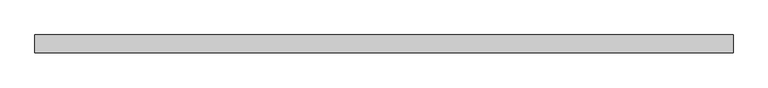
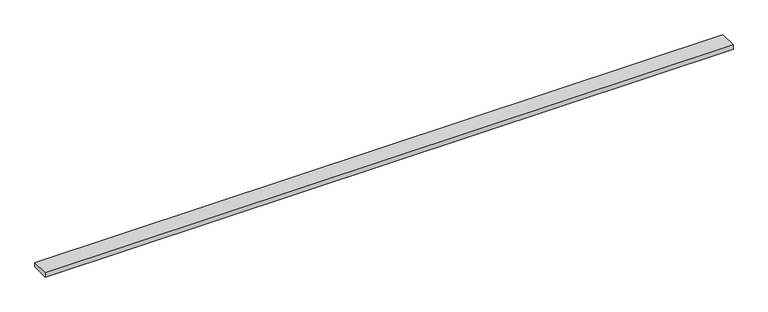
"""IFC4 building model written with IfcOpenShell, lengths in millimetres: proxy geometry, Generic Models 6:Generic Models 2:318829:Generic Models 2:318829 : Generic Models 6:Generic Models 2:318829:20 : Generic Models 6:Generic Models 2:318829:Generic Models 2:318829 : Generic Models 6:Generic Models 2:318829:300683."""

from ifc_helpers import new_model, si_unit, frame, origin, place, context, project, spatial, polyline, outline, extrude, source, transform, mapped, element, save


def generic_models_66336ed3(model_context):
    return source(origin(), model_context, "Body", "SweptSolid", [
        extrude(outline(polyline([(592755.4242239, -579000.6913841), (592755.4242239, -579063.015441), (590317.0242239, -579063.015441), (590317.0242239, -579000.6913841), (592755.4242239, -579000.6913841)])), frame((0.0, 0.0, 3699.7749221), z_axis=(0.0, 0.0, 1.0), x_axis=(1.0, 0.0, 0.0)), (0.0, 0.0, 1.0), 15.837253),
    ])


if __name__ == "__main__":
    model = new_model("IFC4")
    model_context = context("Model", 3, world=origin())
    ifc_project = project(units=[si_unit("LENGTHUNIT", "METRE", prefix="MILLI")], contexts=[model_context])
    site = spatial("IfcSite", under=ifc_project)
    building = spatial("IfcBuilding", under=site)
    placement = place(None, origin())
    generic_models_shape = generic_models_66336ed3(model_context)
    element("IfcBuildingElementProxy", 1, Name="Generic Models 6:Generic Models 2:318829:Generic Models 2:318829 : Generic Models 6:Generic Models 2:318829:20 : Generic Models 6:Generic Models 2:318829:Generic Models 2:318829 : Generic Models 6:Generic Models 2:318829:300683", ObjectType="Generic Models 6:Generic Models 2:318829:Generic Models 2:318829 : Generic Models 6:Generic Models 2:318829:20 : Generic Models 6:Generic Models 2:318829:Generic Models 2:318829 : Generic Models 6:Generic Models 2:318829:300683", at=placement, inside=building, context=model_context, shape_type="MappedRepresentation", body=[
        mapped(generic_models_shape, transform((0.0, 0.0, 0.0), x_axis=(1.0, 0.0, 0.0), y_axis=(0.0, 1.0, 0.0), z_axis=(0.0, 0.0, 1.0))),
    ])
    save(model, "model.ifc")

# Revit data of these elements
# Type "Generic Models 6:Generic Models 2:318829:Generic Models 2:318829 : Generic Models 6:Generic Models 2:318829:20 : Generic Models 6:Generic Models 2:318829:Generic Models 2:318829 : Generic Models 6:Generic Models 2:318829:300683"
#   NameOverride = "Generic Models 6:Generic Models 2:318829:Generic Models 2:318829 : Generic Models 6:Generic Models 2:318829:300683"
#   ObjectTypeOverride = "Generic Models 2:318829 : Generic Models 6:Generic Models 2:318829"
#   Reference = "Generic Models 2"
#   Tag = "300683"
# Element 1 (IfcBuildingElementProxy, "Generic Models 6:Generic Models 2:318829:Generic Models 2:318829 : Generic Models 6:Generic Models 2:318829:20 : Generic Models 6:Generic Models 2:318829:Generic Models 2:318829 : Generic Models 6:Generic Models 2:318829:300683")
#   Materials on its faces: "WOOD BLOCKING - SIZE AS NECESSARY"
# Materials
#   "WOOD BLOCKING - SIZE AS NECESSARY": class "Wood", colour RGB 144 113 62, transparency 0, Description = "Pinus Echinata", Cost = 0
